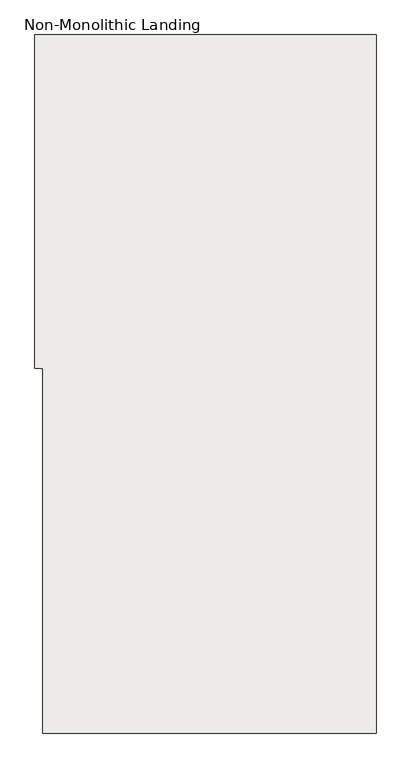
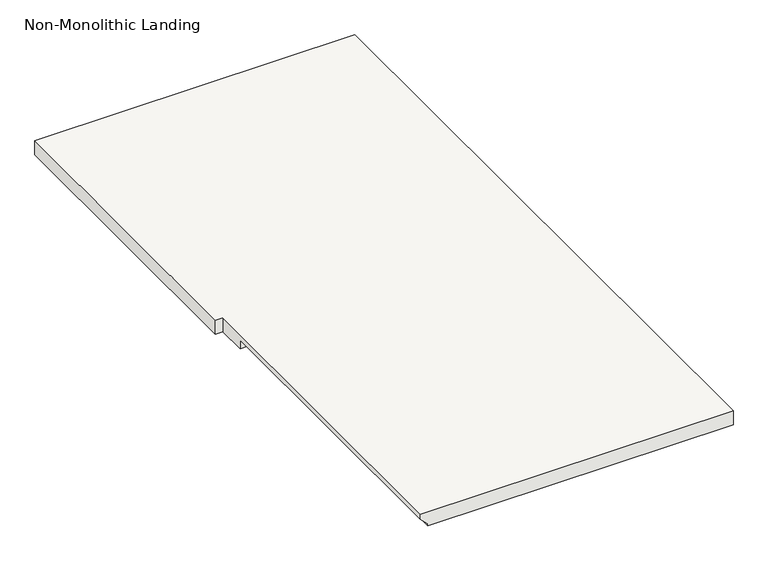
"""IFC4 building model written with IfcOpenShell, lengths in millimetres: slab geometry, Non-Monolithic Landing."""

from ifc_helpers import new_model, si_unit, origin, place, context, project, spatial, faceted_brep, source, transform, mapped, element, save


def non_monolithic_landing_eb16da41(model_context):
    return source(origin(), model_context, "Body", "Brep", [
        faceted_brep([(665981.788677, -551651.2413841, 3291.8743243), (665956.388677, -551651.2413841, 3317.2743243), (665956.388677, -550584.4413841, 3317.2743243), (665981.788677, -550584.4413841, 3291.8743243), (667023.188677, -551651.2413841, 3336.3243243), (667023.188677, -549416.0413841, 3336.3243243), (665956.388677, -549416.0413841, 3336.3243243), (665930.988677, -549416.0413841, 3336.3243243), (665930.988677, -550482.8413841, 3336.3243243), (665956.388677, -550482.8413841, 3336.3243243), (665956.388677, -551651.2413841, 3336.3243243), (665981.788677, -550584.4413841, 3285.5243243), (665956.388677, -550584.4413841, 3285.5243243), (665956.388677, -550482.8413841, 3285.5243243), (665930.988677, -550482.8413841, 3285.5243243), (665930.988677, -549416.0413841, 3285.5243243), (665956.388677, -549416.0413841, 3285.5243243), (667023.188677, -549416.0413841, 3285.5243243), (667023.188677, -551651.2413841, 3285.5243243), (665981.788677, -551651.2413841, 3285.5243243)], [[[0, 1, 2, 3]], [[4, 5, 6, 7, 8, 9, 10]], [[11, 12, 13, 14, 15, 16, 17, 18, 19]], [[12, 11, 3, 2]], [[11, 19, 0, 3]], [[4, 10, 1, 0, 19, 18]], [[5, 4, 18, 17]], [[6, 5, 17, 16]], [[7, 6, 16, 15]], [[8, 7, 15, 14]], [[9, 8, 14, 13]], [[10, 9, 13, 12, 2, 1]]]),
    ])


if __name__ == "__main__":
    model = new_model("IFC4")
    model_context = context("Model", 3, world=origin())
    ifc_project = project(units=[si_unit("LENGTHUNIT", "METRE", prefix="MILLI")], contexts=[model_context])
    site = spatial("IfcSite", under=ifc_project)
    building = spatial("IfcBuilding", under=site)
    placement = place(None, origin())
    non_monolithic_landing_shape = non_monolithic_landing_eb16da41(model_context)
    element("IfcSlab", 1, ObjectType="Non-Monolithic Landing", at=placement, inside=building, context=model_context, shape_type="MappedRepresentation", body=[
        mapped(non_monolithic_landing_shape, transform((0.0, 0.0, 0.0), x_axis=(1.0, 0.0, 0.0), y_axis=(0.0, 1.0, 0.0), z_axis=(0.0, 0.0, 1.0))),
    ])
    save(model, "model.ifc")
